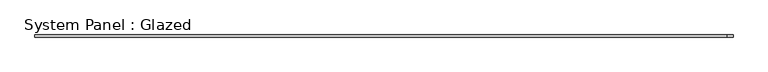
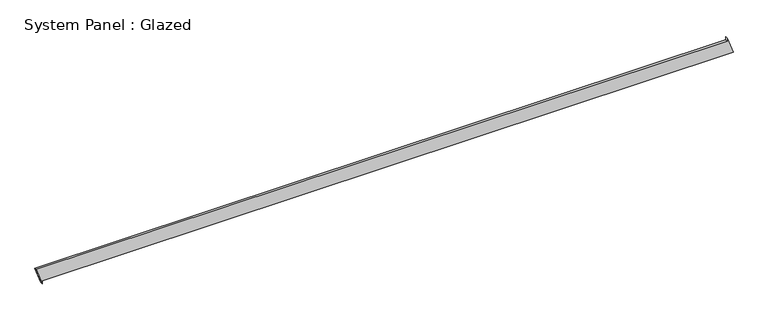
"""IFC4 building model written with IfcOpenShell, lengths in millimetres: plate geometry, System Panel : Glazed."""

from ifc_helpers import new_model, si_unit, frame, origin, place, context, project, spatial, polyline, outline, extrude, source, transform, mapped, element, save


def system_panel_glazed_ae9a7b9e(model_context):
    return source(origin(), model_context, "Body", "SweptSolid", [
        extrude(outline(polyline([(0.0, -3958.3929013), (35.3553391, -3958.3929013), (35.3553391, 4028.5329041), (235.1902238, 3958.4993271), (199.8348847, 3958.4995256), (199.7900514, -4028.5329041), (0.0, -3958.3929013)])), frame((0.0, -49.5, 0.0), z_axis=(0.0, 1.0, 0.0), x_axis=(0.0, 0.0, 1.0)), (0.0, 0.0, 1.0), 25.0),
    ])


if __name__ == "__main__":
    model = new_model("IFC4")
    model_context = context("Model", 3, world=origin())
    ifc_project = project(units=[si_unit("LENGTHUNIT", "METRE", prefix="MILLI")], contexts=[model_context])
    site = spatial("IfcSite", under=ifc_project)
    building = spatial("IfcBuilding", under=site)
    placement = place(None, origin())
    system_panel_glazed_shape = system_panel_glazed_ae9a7b9e(model_context)
    element("IfcPlate", 1, ObjectType="System Panel : Glazed", at=placement, inside=building, context=model_context, shape_type="MappedRepresentation", body=[
        mapped(system_panel_glazed_shape, transform((0.0, 0.0, 0.0), x_axis=(1.0, 0.0, 0.0), y_axis=(0.0, 1.0, 0.0), z_axis=(0.0, 0.0, 1.0))),
    ])
    save(model, "model.ifc")

# Revit data of these elements
# Element 1 (IfcPlate, "System Panel : Glazed")
#   Materials on its faces: "Glass"
# Materials
#   "Glass": class "Glass", colour RGB 218 227 224, transparency 0.85, Description = "Soda Lime Glass", Cost = 0
